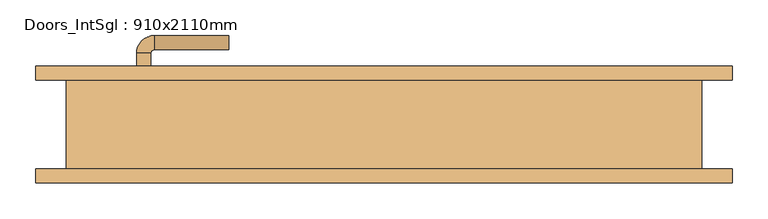
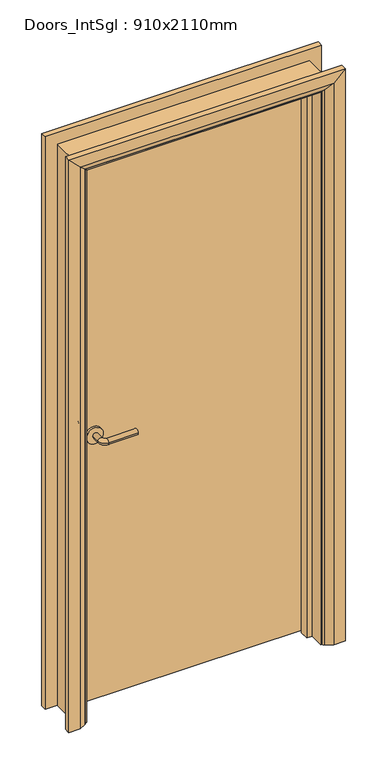
"""IFC4 building model written with IfcOpenShell, lengths in millimetres: door geometry, Doors_IntSgl : 910x2110mm."""

import ifcopenshell
import ifcopenshell.guid

model = None  # the IFC model being written
_history = None  # IfcOwnerHistory: only IFC2X3 demands one
_inside = {}  # id of a spatial element -> (the spatial element, [elements in it])
_under = {}  # id of a project, library or spatial element -> (it, [spatial elements below it])
_declared = {}  # id of a project -> (the project, [libraries it declares])
_typed = {}  # id of a type object -> (the type object, [elements of that type])
_made_of = {}  # id of a material, layer set ... -> (it, [elements and type objects made of it])


def new_model(schema):
    """Start an empty IFC model of exactly this schema.

    Asked for "IFC4X3", IfcOpenShell would pick the latest addendum, in which some entities
    have other attributes; the version numbers below select the first issue.
    IFC2X3 requires an IfcOwnerHistory on every rooted entity: one is made here for all.
    """
    global model, _history
    if schema == "IFC4X3":
        model = ifcopenshell.file(schema_version=(4, 3, 0, 0))
    else:
        model = ifcopenshell.file(schema=schema)
    _inside.clear()
    _under.clear()
    _declared.clear()
    _typed.clear()
    _made_of.clear()
    _history = None
    if model.schema == "IFC2X3":
        org = make("IfcOrganization", Name="unknown")
        user = make(
            "IfcPersonAndOrganization",
            ThePerson=make("IfcPerson", FamilyName="unknown"),
            TheOrganization=org,
        )
        app = make(
            "IfcApplication",
            ApplicationDeveloper=org,
            Version="unknown",
            ApplicationFullName="unknown",
            ApplicationIdentifier="unknown",
        )
        _history = make(
            "IfcOwnerHistory",
            OwningUser=user,
            OwningApplication=app,
            ChangeAction="ADDED",
            CreationDate=0,
        )
    return model


def make(cls, **values):
    """One entity of the class cls with the attributes given. An attribute that is None is left unset."""
    return model.create_entity(
        cls, **{name: value for name, value in values.items() if value is not None}
    )


def rooted(cls, **values):
    """An entity with a GlobalId (a new one), such as an element, a storey or a relation."""
    return make(cls, GlobalId=ifcopenshell.guid.new(), OwnerHistory=_history, **values)


def si_unit(unit_type, name, prefix=None):
    """IfcSIUnit, for example si_unit("LENGTHUNIT", "METRE", prefix="MILLI")."""
    return make("IfcSIUnit", UnitType=unit_type, Prefix=prefix, Name=name)


def assignment(units):
    """IfcUnitAssignment: the units of a project."""
    return None if units is None else make("IfcUnitAssignment", Units=units)


def point(xyz):
    """IfcCartesianPoint."""
    return None if xyz is None else make("IfcCartesianPoint", Coordinates=xyz)


def direction(xyz):
    """IfcDirection."""
    return None if xyz is None else make("IfcDirection", DirectionRatios=xyz)


def frame(location, z_axis=None, x_axis=None):
    """IfcAxis2Placement3D, a coordinate frame: its origin and axes. An axis left out is left unset."""
    return make(
        "IfcAxis2Placement3D",
        Location=point(location),
        Axis=direction(z_axis),
        RefDirection=direction(x_axis),
    )


def frame_2d(location, x_axis=None):
    """IfcAxis2Placement2D, a coordinate frame in the plane: its origin and x axis."""
    return make(
        "IfcAxis2Placement2D", Location=point(location), RefDirection=direction(x_axis)
    )


def origin():
    """The frame at (0, 0, 0) with its axes left unset."""
    return frame((0.0, 0.0, 0.0))


def place(relative_to, where):
    """IfcLocalPlacement: puts the frame where relative to a parent placement (None: the world)."""
    return make(
        "IfcLocalPlacement", PlacementRelTo=relative_to, RelativePlacement=where
    )


def context(
    kind, dimensions, precision=None, world=None, true_north=None, identifier=None
):
    """IfcGeometricRepresentationContext, for example the 3D "Model" context."""
    return make(
        "IfcGeometricRepresentationContext",
        ContextIdentifier=identifier,
        ContextType=kind,
        CoordinateSpaceDimension=dimensions,
        Precision=precision,
        WorldCoordinateSystem=world,
        TrueNorth=true_north,
    )


def project(units=None, contexts=None):
    """IfcProject with its units and contexts."""
    return rooted(
        "IfcProject",
        Name="project",
        RepresentationContexts=contexts,
        UnitsInContext=assignment(units),
    )


def spatial(cls, under=None, at=None, **own):
    """A site, building, storey or space (cls), placed at a placement, below another one or the project."""
    s = rooted(cls, ObjectPlacement=at, **own)
    if under is not None:
        _under.setdefault(under.id(), (under, []))[1].append(s)
    return s


def polyline(points):
    """IfcPolyline through the points."""
    return make("IfcPolyline", Points=[point(p) for p in points])


def circle_curve(where, radius):
    """IfcCircle in the frame where."""
    return make("IfcCircle", Position=where, Radius=radius)


def ellipse_curve(where, semi_axis1, semi_axis2):
    """IfcEllipse in the frame where."""
    return make(
        "IfcEllipse", Position=where, SemiAxis1=semi_axis1, SemiAxis2=semi_axis2
    )


def trimmed(basis, trim1, trim2, sense, master):
    """IfcTrimmedCurve: the piece of a basis curve between two trims."""
    return make(
        "IfcTrimmedCurve",
        BasisCurve=basis,
        Trim1=trim1,
        Trim2=trim2,
        SenseAgreement=sense,
        MasterRepresentation=master,
    )


def segment(curve, same_sense, transition):
    """IfcCompositeCurveSegment."""
    return make(
        "IfcCompositeCurveSegment",
        Transition=transition,
        SameSense=same_sense,
        ParentCurve=curve,
    )


def composite_curve(segments, self_intersect=None):
    """IfcCompositeCurve: segments joined end to end."""
    return make("IfcCompositeCurve", Segments=segments, SelfIntersect=self_intersect)


def outline(outer, holes=None, kind="AREA"):
    """IfcArbitraryClosedProfileDef: a profile drawn as a closed curve; with holes, ...WithVoids."""
    if holes is None:
        return make("IfcArbitraryClosedProfileDef", ProfileType=kind, OuterCurve=outer)
    return make(
        "IfcArbitraryProfileDefWithVoids",
        ProfileType=kind,
        OuterCurve=outer,
        InnerCurves=holes,
    )


def extrude(swept, where, along, depth):
    """IfcExtrudedAreaSolid: the profile swept, set in the frame where, extruded along a direction by depth."""
    return make(
        "IfcExtrudedAreaSolid",
        SweptArea=swept,
        Position=where,
        ExtrudedDirection=direction(along),
        Depth=depth,
    )


def faces_of(points, faces, orient=None, outer=None):
    """IfcFace entities. A face is a list of loops; a loop is a list of indices into points, from 0.

    orient and outer hold one flag for each loop. By default every Orientation is true, the
    first loop of a face is its IfcFaceOuterBound and the others are IfcFaceBound.
    """
    made = []
    for i, loops in enumerate(faces):
        bounds = []
        for j, loop in enumerate(loops):
            is_outer = j == 0 if outer is None else outer[i][j]
            bounds.append(
                make(
                    "IfcFaceOuterBound" if is_outer else "IfcFaceBound",
                    Bound=make("IfcPolyLoop", Polygon=[points[k] for k in loop]),
                    Orientation=True if orient is None else orient[i][j],
                )
            )
        made.append(make("IfcFace", Bounds=bounds))
    return made


def faceted_brep(points, faces, orient=None, outer=None, voids=None):
    """IfcFacetedBrep: a solid bounded by flat faces; with voids (closed shells), ...WithVoids."""
    shared = [point(p) for p in points]
    hull = make("IfcClosedShell", CfsFaces=faces_of(shared, faces, orient, outer))
    if voids is None:
        return make("IfcFacetedBrep", Outer=hull)
    return make(
        "IfcFacetedBrepWithVoids",
        Outer=hull,
        Voids=[
            make(cls, CfsFaces=faces_of(shared, fs, o, b)) for cls, fs, o, b in voids
        ],
    )


def shape(context_of_items, identifier, shape_type, items):
    """IfcShapeRepresentation: the items that make up one representation, for example the "Body"."""
    return make(
        "IfcShapeRepresentation",
        ContextOfItems=context_of_items,
        RepresentationIdentifier=identifier,
        RepresentationType=shape_type,
        Items=items,
    )


def source(mapping_origin, context_of_items, identifier, shape_type, items):
    """IfcRepresentationMap: a shape defined once, which mapped items show again and again."""
    return make(
        "IfcRepresentationMap",
        MappingOrigin=mapping_origin,
        MappedRepresentation=shape(context_of_items, identifier, shape_type, items),
    )


def transform(
    local_origin,
    x_axis=None,
    y_axis=None,
    z_axis=None,
    scale=None,
    scale2=None,
    scale3=None,
    uniform=True,
):
    """IfcCartesianTransformationOperator3D, or its non-uniform kind. x_axis, y_axis, z_axis: its Axis1, 2, 3."""
    if uniform:
        return make(
            "IfcCartesianTransformationOperator3D",
            Axis1=direction(x_axis),
            Axis2=direction(y_axis),
            LocalOrigin=point(local_origin),
            Scale=scale,
            Axis3=direction(z_axis),
        )
    return make(
        "IfcCartesianTransformationOperator3DnonUniform",
        Axis1=direction(x_axis),
        Axis2=direction(y_axis),
        LocalOrigin=point(local_origin),
        Scale=scale,
        Axis3=direction(z_axis),
        Scale2=scale2,
        Scale3=scale3,
    )


def mapped(mapping_source, mapping_target):
    """IfcMappedItem: shows the shape of a source again, moved by a transform."""
    return make(
        "IfcMappedItem", MappingSource=mapping_source, MappingTarget=mapping_target
    )


def made_of(thing, what):
    """Note that an element or type object is made of a material, layer set ...; save() writes the relation."""
    if what is not None:
        _made_of.setdefault(what.id(), (what, []))[1].append(thing)
    return thing


def element(
    cls,
    number,
    at=None,
    inside=None,
    cuts=None,
    type_object=None,
    material=None,
    context=None,
    identifier="Body",
    shape_type=None,
    held_by="IfcProductDefinitionShape",
    body=None,
    shapes=None,
    **own,
):
    """One element of the class cls, such as IfcWall. Its Tag is "e" and its number.

    at: its placement. inside: the storey or other place that contains it. cuts: it is an
    opening in that element (IfcRelVoidsElement). A single representation is given by context,
    identifier, shape_type and body (its items); several are given by shapes. held_by: the class
    of the entity that holds the representations. save() writes the other relations.
    """
    e = rooted(cls, Tag="e%d" % number, ObjectPlacement=at, **own)
    if body is not None:
        shapes = [shape(context, identifier, shape_type, body)]
    if shapes is not None:
        e.Representation = make(held_by, Representations=shapes)
    if inside is not None:
        _inside.setdefault(inside.id(), (inside, []))[1].append(e)
    if cuts is not None:
        rooted(
            "IfcRelVoidsElement", RelatingBuildingElement=cuts, RelatedOpeningElement=e
        )
    if type_object is not None:
        _typed.setdefault(type_object.id(), (type_object, []))[1].append(e)
    return made_of(e, material)


def aggregate(whole, parts):
    """IfcRelAggregates: a whole, such as a stair, and the parts it consists of."""
    return rooted("IfcRelAggregates", RelatingObject=whole, RelatedObjects=parts)


def save(model, path):
    """Write the relations noted so far, then the file.

    IfcRelAggregates (storeys below a building ...), IfcRelContainedInSpatialStructure (elements
    in a storey), IfcRelDefinesByType, IfcRelAssociatesMaterial and IfcRelDeclares: one each for
    every whole, place, type object, material and project.
    """
    for whole, parts in _under.values():
        aggregate(whole, parts)
    for where, things in _inside.values():
        rooted(
            "IfcRelContainedInSpatialStructure",
            RelatedElements=things,
            RelatingStructure=where,
        )
    for kind, things in _typed.values():
        rooted("IfcRelDefinesByType", RelatedObjects=things, RelatingType=kind)
    for what, things in _made_of.values():
        rooted("IfcRelAssociatesMaterial", RelatedObjects=things, RelatingMaterial=what)
    for by, libraries in _declared.values():
        rooted("IfcRelDeclares", RelatingContext=by, RelatedDefinitions=libraries)
    model.write(path)


def plane_surface(at):
    """IfcPlane: the flat surface through the origin of the frame at, square to its z axis."""
    return make("IfcPlane", Position=at)


def cylinder_surface(at, radius):
    """IfcCylindricalSurface: all points at the distance radius from the z axis of the frame at."""
    return make("IfcCylindricalSurface", Position=at, Radius=radius)


def revolved_surface(curve, axis_point, axis_direction):
    """IfcSurfaceOfRevolution: the curve turned about the line through axis_point along axis_direction."""
    return make(
        "IfcSurfaceOfRevolution",
        SweptCurve=make("IfcArbitraryOpenProfileDef", ProfileType="CURVE", Curve=curve),
        AxisPosition=make("IfcAxis1Placement", Location=point(axis_point), Axis=direction(axis_direction)),
    )


def advanced_brep(points, edges, surfaces, faces):
    """IfcAdvancedBrep: a solid bounded by faces that lie on surfaces and meet in shared edges.

    An edge is (start, end): straight between two places in points (the first is 0);
    or (start, end, curve); or (start, end, curve, False) where it runs against its curve.
    A face is (place in surfaces, loops), or (place, loops, False) where it looks against
    its surface's normal. A loop lists edges by number (the first is 1), with a minus sign
    where the edge is run from its end to its start. The first loop is the outer one.
    """
    corners = [point(p) for p in points]
    vertices = [make("IfcVertexPoint", VertexGeometry=c) for c in corners]
    made = []
    for start, end, *more in edges:
        made.append(
            make(
                "IfcEdgeCurve",
                EdgeStart=vertices[start],
                EdgeEnd=vertices[end],
                EdgeGeometry=more[0] if more else make("IfcPolyline", Points=[corners[start], corners[end]]),
                SameSense=more[1] if len(more) > 1 else True,
            )
        )
    hull = []
    for where, loops, *sense in faces:
        bounds = []
        for j, loop in enumerate(loops):
            ring = [make("IfcOrientedEdge", EdgeElement=made[abs(k) - 1], Orientation=k > 0) for k in loop]
            bounds.append(
                make(
                    "IfcFaceOuterBound" if j == 0 else "IfcFaceBound",
                    Bound=make("IfcEdgeLoop", EdgeList=ring),
                    Orientation=True,
                )
            )
        hull.append(make("IfcAdvancedFace", Bounds=bounds, FaceSurface=surfaces[where], SameSense=sense[0] if sense else True))
    return make("IfcAdvancedBrep", Outer=make("IfcClosedShell", CfsFaces=hull))


def doors_intsgl_910x2110mm_1208da3b(model_context):
    return source(origin(), model_context, "Body", "SolidModel", [
        advanced_brep(
        [(-348.0, 16.5, 1000.0), (-328.0, 16.5, 1000.0), (-328.0, -13.5, 1000.0), (-348.0, -13.5, 1000.0), (-323.0, -18.5, 1000.0), (-323.0, -38.5, 1000.0), (-218.0, -38.5, 1000.0), (-218.0, -18.5, 1000.0)],
        [
            (0, 1, circle_curve(frame((-338.0, 16.5, 1000.0), z_axis=(0.0, 1.0, 0.0), x_axis=(1.0, 0.0, 0.0)), 10.0)),
            (1, 0, circle_curve(frame((-338.0, 16.5, 1000.0), z_axis=(0.0, 1.0, 0.0), x_axis=(1.0, 0.0, 0.0)), 10.0)),
            (1, 2),
            (2, 3, circle_curve(frame((-338.0, -13.5, 1000.0), z_axis=(0.0, 1.0, 0.0), x_axis=(1.0, 0.0, 0.0)), 10.0)),
            (3, 0),
            (3, 2, circle_curve(frame((-338.0, -13.5, 1000.0), z_axis=(0.0, 1.0, 0.0), x_axis=(1.0, 0.0, 0.0)), 10.0)),
            (4, 5, circle_curve(frame((-323.0, -28.5, 1000.0), z_axis=(-1.0, 0.0, 0.0), x_axis=(0.0, 1.0, 0.0)), 10.0)),
            (5, 3, circle_curve(frame((-323.0, -13.5, 1000.0), z_axis=(0.0, 0.0, -1.0), x_axis=(-1.0, 0.0, 0.0)), 25.0)),
            (2, 4, circle_curve(frame((-323.0, -13.5, 1000.0), z_axis=(0.0, 0.0, 1.0), x_axis=(-1.0, 0.0, 0.0)), 5.0)),
            (5, 4, circle_curve(frame((-323.0, -28.5, 1000.0), z_axis=(-1.0, 0.0, 0.0), x_axis=(0.0, 1.0, 0.0)), 10.0)),
            (6, 7, circle_curve(frame((-218.0, -28.5, 1000.0), z_axis=(1.0, 0.0, 0.0), x_axis=(0.0, 1.0, 0.0)), 10.0)),
            (7, 6, circle_curve(frame((-218.0, -28.5, 1000.0), z_axis=(1.0, 0.0, 0.0), x_axis=(0.0, 1.0, 0.0)), 10.0)),
            (4, 7),
            (6, 5),
        ],
        [
            plane_surface(frame((-338.0, 16.5, 1000.0), z_axis=(0.0, 1.0, 0.0), x_axis=(0.0, 0.0, 1.0))),
            cylinder_surface(frame((-338.0, 16.5, 1000.0), z_axis=(0.0, 1.0, 0.0), x_axis=(1.0, 0.0, 0.0)), 10.0),
            revolved_surface(trimmed(ellipse_curve(frame((-338.0, -13.5, 1000.0), z_axis=(0.0, -1.0, 0.0), x_axis=(1.0, 0.0, 0.0)), 10.0, 10.0), [point((-348.0, -13.5, 1000.0))], [point((-328.0, -13.5, 1000.0))], True, "CARTESIAN"), (-323.0, -13.5, 1000.0), (0.0, 0.0, -1.0)),
            revolved_surface(trimmed(ellipse_curve(frame((-338.0, -13.5, 1000.0), z_axis=(0.0, -1.0, 0.0), x_axis=(1.0, 0.0, 0.0)), 10.0, 10.0), [point((-328.0, -13.5, 1000.0))], [point((-348.0, -13.5, 1000.0))], True, "CARTESIAN"), (-323.0, -13.5, 1000.0), (0.0, 0.0, -1.0)),
            plane_surface(frame((-218.0, -28.5, 1000.0), z_axis=(1.0, 0.0, 0.0), x_axis=(0.0, 0.0, 1.0))),
            cylinder_surface(frame((-323.0, -28.5, 1000.0), z_axis=(-1.0, 0.0, 0.0), x_axis=(0.0, 1.0, 0.0)), 10.0),
        ],
        [
            (0, [[1, 2]]),
            (1, [[3, 4, 5, -2]]),
            (1, [[-5, 6, -3, -1]]),
            (2, [[7, 8, -4, 9]]),
            (3, [[10, -9, -6, -8]]),
            (4, [[11, 12]]),
            (5, [[13, -11, 14, -7]]),
            (5, [[-14, -12, -13, -10]]),
        ],
    ),
        extrude(outline(composite_curve([segment(trimmed(circle_curve(frame_2d((1000.0, -340.5)), 30.0), [point((1000.0, -370.5))], [point((1000.0, -310.5))], False, "CARTESIAN"), True, "CONTINUOUS"), segment(trimmed(circle_curve(frame_2d((1000.0, -340.5)), 30.0), [point((1000.0, -310.5))], [point((1000.0, -370.5))], False, "CARTESIAN"), True, "CONTINUOUS")], self_intersect=False)), frame((0.0, 16.5, 0.0), z_axis=(0.0, 1.0, 0.0), x_axis=(0.0, 0.0, 1.0)), (0.0, 0.0, 1.0), 8.0),
        advanced_brep(
        [(-348.0, 70.5, 1000.0), (-328.0, 70.5, 1000.0), (-348.0, 100.5, 1000.0), (-328.0, 100.5, 1000.0), (-323.0, 105.5, 1000.0), (-323.0, 125.5, 1000.0), (-218.0, 125.5, 1000.0), (-218.0, 105.5, 1000.0)],
        [
            (0, 1, circle_curve(frame((-338.0, 70.5, 1000.0), z_axis=(0.0, -1.0, 0.0), x_axis=(1.0, 0.0, 0.0)), 10.0)),
            (1, 0, circle_curve(frame((-338.0, 70.5, 1000.0), z_axis=(0.0, -1.0, 0.0), x_axis=(1.0, 0.0, 0.0)), 10.0)),
            (0, 2),
            (2, 3, circle_curve(frame((-338.0, 100.5, 1000.0), z_axis=(0.0, -1.0, 0.0), x_axis=(1.0, 0.0, 0.0)), 10.0)),
            (3, 1),
            (3, 2, circle_curve(frame((-338.0, 100.5, 1000.0), z_axis=(0.0, -1.0, 0.0), x_axis=(1.0, 0.0, 0.0)), 10.0)),
            (4, 3, circle_curve(frame((-323.0, 100.5, 1000.0), z_axis=(0.0, 0.0, 1.0), x_axis=(-1.0, 0.0, 0.0)), 5.0)),
            (2, 5, circle_curve(frame((-323.0, 100.5, 1000.0), z_axis=(0.0, 0.0, -1.0), x_axis=(-1.0, 0.0, 0.0)), 25.0)),
            (5, 4, circle_curve(frame((-323.0, 115.5, 1000.0), z_axis=(-1.0, 0.0, 0.0), x_axis=(0.0, -1.0, 0.0)), 10.0)),
            (4, 5, circle_curve(frame((-323.0, 115.5, 1000.0), z_axis=(-1.0, 0.0, 0.0), x_axis=(0.0, -1.0, 0.0)), 10.0)),
            (6, 7, circle_curve(frame((-218.0, 115.5, 1000.0), z_axis=(1.0, 0.0, 0.0), x_axis=(0.0, -1.0, 0.0)), 10.0)),
            (7, 6, circle_curve(frame((-218.0, 115.5, 1000.0), z_axis=(1.0, 0.0, 0.0), x_axis=(0.0, -1.0, 0.0)), 10.0)),
            (5, 6),
            (7, 4),
        ],
        [
            plane_surface(frame((-338.0, 70.5, 1000.0), z_axis=(0.0, -1.0, 0.0), x_axis=(0.0, 0.0, 1.0))),
            cylinder_surface(frame((-338.0, 70.5, 1000.0), z_axis=(0.0, -1.0, 0.0), x_axis=(1.0, 0.0, 0.0)), 10.0),
            revolved_surface(trimmed(ellipse_curve(frame((-338.0, 100.5, 1000.0), z_axis=(0.0, -1.0, 0.0), x_axis=(1.0, 0.0, 0.0)), 10.0, 10.0), [point((-348.0, 100.5, 1000.0))], [point((-328.0, 100.5, 1000.0))], True, "CARTESIAN"), (-323.0, 100.5, 1000.0), (0.0, 0.0, -1.0)),
            revolved_surface(trimmed(ellipse_curve(frame((-338.0, 100.5, 1000.0), z_axis=(0.0, -1.0, 0.0), x_axis=(1.0, 0.0, 0.0)), 10.0, 10.0), [point((-328.0, 100.5, 1000.0))], [point((-348.0, 100.5, 1000.0))], True, "CARTESIAN"), (-323.0, 100.5, 1000.0), (0.0, 0.0, -1.0)),
            plane_surface(frame((-218.0, 115.5, 1000.0), z_axis=(1.0, 0.0, 0.0), x_axis=(0.0, 0.0, 1.0))),
            cylinder_surface(frame((-323.0, 115.5, 1000.0), z_axis=(-1.0, 0.0, 0.0), x_axis=(0.0, -1.0, 0.0)), 10.0),
        ],
        [
            (0, [[1, 2]]),
            (1, [[-1, 3, 4, 5]]),
            (1, [[-2, -5, 6, -3]]),
            (2, [[7, -4, 8, 9]]),
            (3, [[-8, -6, -7, 10]]),
            (4, [[11, 12]]),
            (5, [[-9, 13, -12, 14]]),
            (5, [[-10, -14, -11, -13]]),
        ],
    ),
        extrude(outline(composite_curve([segment(trimmed(circle_curve(frame_2d((1000.0, -340.5)), 30.0), [point((1000.0, -370.5))], [point((1000.0, -310.5))], False, "CARTESIAN"), True, "CONTINUOUS"), segment(trimmed(circle_curve(frame_2d((1000.0, -340.5)), 30.0), [point((1000.0, -310.5))], [point((1000.0, -370.5))], False, "CARTESIAN"), True, "CONTINUOUS")], self_intersect=False)), frame((0.0, 62.5, 0.0), z_axis=(0.0, 1.0, 0.0), x_axis=(0.0, 0.0, 1.0)), (0.0, 0.0, 1.0), 8.0),
        extrude(outline(polyline([(413.0, 24.5), (-413.0, 24.5), (-413.0, 62.5), (413.0, 62.5), (413.0, 24.5)])), frame((0.0, 0.0, 8.0), z_axis=(0.0, 0.0, 1.0), x_axis=(1.0, 0.0, 0.0)), (0.0, 0.0, 1.0), 2060.0),
        advanced_brep(
        [(490.0, 82.5, 0.0), (490.0, 62.5, 0.0), (420.0, 62.5, 0.0), (424.0, 68.5, 0.0), (450.0, 82.5, 0.0), (490.0, 82.5, 2145.0), (490.0, 62.5, 2145.0), (-490.0, 62.5, 2145.0), (-490.0, 62.5, 0.0), (-420.0, 62.5, 0.0), (-420.0, 62.5, 2075.0), (420.0, 62.5, 2075.0), (424.0, 68.5, 2079.0), (450.0, 82.5, 2105.0), (-450.0, 82.5, 2105.0), (-450.0, 82.5, 0.0), (-490.0, 82.5, 0.0), (-490.0, 82.5, 2145.0), (-424.0, 68.5, 2079.0), (-424.0, 68.5, 0.0)],
        [
            (0, 1),
            (1, 2),
            (2, 3, circle_curve(frame((428.0, 61.5, 0.0), z_axis=(0.0, 0.0, -1.0), x_axis=(1.0, 0.0, 0.0)), 8.0622577)),
            (3, 4),
            (4, 0),
            (0, 5),
            (5, 6),
            (6, 1),
            (6, 7),
            (7, 8),
            (8, 9),
            (9, 10),
            (10, 11),
            (11, 2),
            (11, 12, ellipse_curve(frame((428.0, 61.5, 2083.0), z_axis=(0.7071067811865475, 0.0, -0.7071067811865475), x_axis=(-0.7071067811865474, 0.0, -0.7071067811865476)), 11.4017543, 8.0622577)),
            (12, 3),
            (12, 13),
            (13, 4),
            (13, 14),
            (14, 15),
            (15, 16),
            (16, 17),
            (17, 5),
            (17, 7),
            (10, 18, ellipse_curve(frame((-428.0, 61.5, 2083.0), z_axis=(0.7071067811865475, 0.0, 0.7071067811865475), x_axis=(0.7071067811865476, 0.0, -0.7071067811865474)), 11.4017543, 8.0622577)),
            (18, 12),
            (18, 14),
            (15, 19),
            (19, 9, circle_curve(frame((-428.0, 61.5, 0.0), z_axis=(0.0, 0.0, -1.0), x_axis=(-1.0, 0.0, 0.0)), 8.0622577)),
            (8, 16),
            (19, 18),
        ],
        [
            plane_surface(frame((420.0, 62.5, 0.0), z_axis=(0.0, 0.0, -1.0), x_axis=(0.0, -1.0, 0.0))),
            plane_surface(frame((490.0, 82.5, 0.0), z_axis=(1.0, 0.0, 0.0), x_axis=(0.0, 0.0, 1.0))),
            plane_surface(frame((490.0, 62.5, 0.0), z_axis=(0.0, -1.0, 0.0), x_axis=(0.0, 0.0, 1.0))),
            cylinder_surface(frame((428.0, 61.5, 0.0), z_axis=(0.0, 0.0, -1.0), x_axis=(1.0, 0.0, 0.0)), 8.0622577),
            plane_surface(frame((424.0, 68.5, 0.0), z_axis=(-0.4740998230350126, 0.880471099922178, 0.0), x_axis=(0.0, 0.0, 1.0))),
            plane_surface(frame((450.0, 82.5, 0.0), z_axis=(0.0, 1.0, 0.0), x_axis=(0.0, 0.0, 1.0))),
            plane_surface(frame((490.0, 82.5, 2145.0), z_axis=(0.0, 0.0, 1.0), x_axis=(-1.0, 0.0, 0.0))),
            cylinder_surface(frame((420.0, 61.5, 2083.0), z_axis=(1.0, 0.0, 0.0), x_axis=(0.0, 0.0, 1.0)), 8.0622577),
            plane_surface(frame((424.0, 68.5, 2079.0), z_axis=(0.0, 0.8804710999221764, -0.4740998230350154), x_axis=(-1.0, 0.0, 0.0))),
            plane_surface(frame((-420.0, 62.5, 0.0), z_axis=(0.0, 0.0, -1.0), x_axis=(0.0, -1.0, 0.0))),
            plane_surface(frame((-490.0, 82.5, 2145.0), z_axis=(-1.0, 0.0, 0.0), x_axis=(0.0, 0.0, -1.0))),
            cylinder_surface(frame((-428.0, 61.5, 2075.0), z_axis=(0.0, 0.0, 1.0), x_axis=(-1.0, 0.0, 0.0)), 8.0622577),
            plane_surface(frame((-424.0, 68.5, 2079.0), z_axis=(0.47409982303501824, 0.8804710999221749, 0.0), x_axis=(0.0, 0.0, -1.0))),
        ],
        [
            (0, [[1, 2, 3, 4, 5]]),
            (1, [[-1, 6, 7, 8]]),
            (2, [[-2, -8, 9, 10, 11, 12, 13, 14]]),
            (3, [[-3, -14, 15, 16]]),
            (4, [[-4, -16, 17, 18]]),
            (5, [[-5, -18, 19, 20, 21, 22, 23, -6]]),
            (6, [[-7, -23, 24, -9]]),
            (7, [[-15, -13, 25, 26]]),
            (8, [[-17, -26, 27, -19]]),
            (9, [[-21, 28, 29, -11, 30]]),
            (10, [[-24, -22, -30, -10]]),
            (11, [[-25, -12, -29, 31]]),
            (12, [[-27, -31, -28, -20]]),
        ],
    ),
        extrude(outline(polyline([(0.0, -415.0), (0.0, -396.0), (2051.0, -396.0), (2051.0, 396.0), (0.0, 396.0), (0.0, 415.0), (2070.0, 415.0), (2070.0, -415.0), (0.0, -415.0)])), frame((0.0, -9.5, 0.0), z_axis=(0.0, 1.0, 0.0), x_axis=(0.0, 0.0, 1.0)), (0.0, 0.0, 1.0), 32.0),
        advanced_brep(
        [(-490.0, -82.5, 0.0), (-490.0, -62.5, 0.0), (-420.0, -62.5, 0.0), (-424.0, -68.5, 0.0), (-450.0, -82.5, 0.0), (-490.0, -82.5, 2145.0), (-490.0, -62.5, 2145.0), (-420.0, -62.5, 2075.0), (-424.0, -68.5, 2079.0), (-450.0, -82.5, 2105.0), (490.0, -82.5, 2145.0), (490.0, -62.5, 2145.0), (420.0, -62.5, 2075.0), (424.0, -68.5, 2079.0), (450.0, -82.5, 2105.0), (490.0, -82.5, 0.0), (450.0, -82.5, 0.0), (424.0, -68.5, 0.0), (420.0, -62.5, 0.0), (490.0, -62.5, 0.0)],
        [
            (0, 1),
            (1, 2),
            (2, 3, circle_curve(frame((-428.0, -61.5, 0.0), z_axis=(0.0, 0.0, -1.0), x_axis=(-1.0, 0.0, 0.0)), 8.0622577)),
            (3, 4),
            (4, 0),
            (0, 5),
            (5, 6),
            (6, 1),
            (6, 7),
            (7, 2),
            (7, 8, ellipse_curve(frame((-428.0, -61.5, 2083.0), z_axis=(-0.7071067811865475, 0.0, -0.7071067811865475), x_axis=(0.7071067811865474, 0.0, -0.7071067811865476)), 11.4017543, 8.0622577)),
            (8, 3),
            (8, 9),
            (9, 4),
            (9, 5),
            (5, 10),
            (10, 11),
            (11, 6),
            (11, 12),
            (12, 7),
            (12, 13, ellipse_curve(frame((428.0, -61.5, 2083.0), z_axis=(-0.7071067811865475, 0.0, 0.7071067811865475), x_axis=(-0.7071067811865476, 0.0, -0.7071067811865474)), 11.4017543, 8.0622577)),
            (13, 8),
            (13, 14),
            (14, 9),
            (14, 10),
            (15, 16),
            (16, 17),
            (17, 18, circle_curve(frame((428.0, -61.5, 0.0), z_axis=(0.0, 0.0, -1.0), x_axis=(1.0, 0.0, 0.0)), 8.0622577)),
            (18, 19),
            (19, 15),
            (10, 15),
            (19, 11),
            (18, 12),
            (17, 13),
            (16, 14),
        ],
        [
            plane_surface(frame((-420.0, -135.3010989, 0.0), z_axis=(0.0, 0.0, -1.0), x_axis=(1.0, 0.0, 0.0))),
            plane_surface(frame((-490.0, -82.5, 0.0), z_axis=(-1.0, 0.0, 0.0), x_axis=(0.0, 0.0, 1.0))),
            plane_surface(frame((-490.0, -62.5, 0.0), z_axis=(0.0, 1.0, 0.0), x_axis=(0.0, 0.0, 1.0))),
            cylinder_surface(frame((-428.0, -61.5, 0.0), z_axis=(0.0, 0.0, -1.0), x_axis=(-1.0, 0.0, 0.0)), 8.0622577),
            plane_surface(frame((-424.0, -68.5, 0.0), z_axis=(0.4740998230350183, -0.8804710999221749, 0.0), x_axis=(0.0, 0.0, 1.0))),
            plane_surface(frame((-450.0, -82.5, 0.0), z_axis=(0.0, -1.0, 0.0), x_axis=(0.0, 0.0, 1.0))),
            plane_surface(frame((-490.0, -82.5, 2145.0), z_axis=(0.0, 0.0, 1.0), x_axis=(1.0, 0.0, 0.0))),
            plane_surface(frame((-490.0, -62.5, 2145.0), z_axis=(0.0, 1.0, 0.0), x_axis=(1.0, 0.0, 0.0))),
            cylinder_surface(frame((-420.0, -61.5, 2083.0), z_axis=(-1.0, 0.0, 0.0), x_axis=(0.0, 0.0, 1.0)), 8.0622577),
            plane_surface(frame((-424.0, -68.5, 2079.0), z_axis=(0.0, -0.8804710999221749, -0.4740998230350183), x_axis=(1.0, 0.0, 0.0))),
            plane_surface(frame((-450.0, -82.5, 2105.0), z_axis=(0.0, -1.0, 0.0), x_axis=(1.0, 0.0, 0.0))),
            plane_surface(frame((420.0, -135.3010989, 0.0), z_axis=(0.0, 0.0, -1.0), x_axis=(-1.0, 0.0, 0.0))),
            plane_surface(frame((490.0, -82.5, 2145.0), z_axis=(1.0, 0.0, 0.0), x_axis=(0.0, 0.0, -1.0))),
            plane_surface(frame((490.0, -62.5, 2145.0), z_axis=(0.0, 1.0, 0.0), x_axis=(0.0, 0.0, -1.0))),
            cylinder_surface(frame((428.0, -61.5, 2075.0), z_axis=(0.0, 0.0, 1.0), x_axis=(1.0, 0.0, 0.0)), 8.0622577),
            plane_surface(frame((424.0, -68.5, 2079.0), z_axis=(-0.4740998230350183, -0.8804710999221749, 0.0), x_axis=(0.0, 0.0, -1.0))),
            plane_surface(frame((450.0, -82.5, 2105.0), z_axis=(0.0, -1.0, 0.0), x_axis=(0.0, 0.0, -1.0))),
        ],
        [
            (0, [[1, 2, 3, 4, 5]]),
            (1, [[-1, 6, 7, 8]]),
            (2, [[-2, -8, 9, 10]]),
            (3, [[-3, -10, 11, 12]]),
            (4, [[-4, -12, 13, 14]]),
            (5, [[-5, -14, 15, -6]]),
            (6, [[-7, 16, 17, 18]]),
            (7, [[-9, -18, 19, 20]]),
            (8, [[-11, -20, 21, 22]]),
            (9, [[-13, -22, 23, 24]]),
            (10, [[-15, -24, 25, -16]]),
            (11, [[26, 27, 28, 29, 30]]),
            (12, [[-17, 31, -30, 32]]),
            (13, [[-19, -32, -29, 33]]),
            (14, [[-21, -33, -28, 34]]),
            (15, [[-23, -34, -27, 35]]),
            (16, [[-25, -35, -26, -31]]),
        ],
    ),
        faceted_brep([(-415.0, 62.5, 0.0), (-415.0, -62.5, 0.0), (-447.0, -62.5, 0.0), (-447.0, 62.5, 0.0), (-415.0, 62.5, 2070.0), (-415.0, -62.5, 2070.0), (-447.0, -62.5, 2102.0), (-447.0, 62.5, 2102.0), (415.0, 62.5, 2070.0), (415.0, -62.5, 2070.0), (447.0, -62.5, 2102.0), (447.0, 62.5, 2102.0), (415.0, 62.5, 0.0), (447.0, 62.5, 0.0), (447.0, -62.5, 0.0), (415.0, -62.5, 0.0)], [[[0, 1, 2, 3]], [[1, 0, 4, 5]], [[2, 1, 5, 6]], [[3, 2, 6, 7]], [[0, 3, 7, 4]], [[5, 4, 8, 9]], [[6, 5, 9, 10]], [[7, 6, 10, 11]], [[4, 7, 11, 8]], [[12, 13, 14, 15]], [[9, 8, 12, 15]], [[10, 9, 15, 14]], [[11, 10, 14, 13]], [[8, 11, 13, 12]]]),
    ])


if __name__ == "__main__":
    model = new_model("IFC4")
    model_context = context("Model", 3, world=origin())
    ifc_project = project(units=[si_unit("LENGTHUNIT", "METRE", prefix="MILLI")], contexts=[model_context])
    site = spatial("IfcSite", under=ifc_project)
    building = spatial("IfcBuilding", under=site)
    placement = place(None, origin())
    doors_intsgl_910x2110mm_shape = doors_intsgl_910x2110mm_1208da3b(model_context)
    element("IfcDoor", 1, ObjectType="Doors_IntSgl : 910x2110mm", at=placement, inside=building, context=model_context, shape_type="MappedRepresentation", body=[
        mapped(doors_intsgl_910x2110mm_shape, transform((0.0, 0.0, 0.0), x_axis=(1.0, 0.0, 0.0), y_axis=(0.0, 1.0, 0.0), z_axis=(0.0, 0.0, 1.0))),
    ])
    save(model, "model.ifc")

# Revit data of these elements
# Project information
#   Project Issue Date = "Issue Date"
#   Project Status = "Project Status"
#   Client Name = "PM & BIM"
#   Project Address = "Enter address here"
#   Project Name = "Assignment 1"
#   Project Number = "Project Number"
# Type "Doors_IntSgl : 910x2110mm"
#   Construction Type Id = "MDOOR"
#   Type Mark = "41"
#   Type Comments = "Internal Single"
#   Operation = "SingleSwingRight"
#   Manufacturer = "Revit"
#   Keynote = "L20"
#   Description = "Internal Single Door"
#   Analytic Construction = "Metal"
#   UnderCut = 8 mm
#   Tolerance = 2 mm
#   Thickness = 38 mm
#   Thermal Resistance (R) = 0.270117 (m²·K)/W
#   Structural Tolerance = 8 mm
#   StopDepth = 32 mm
#   Stop Thickness = 19 mm
#   Rough Width = 910 mm
#   Rough Height = 2110 mm
#   Height to Top Lock Rail = 1000 mm
#   Heat Transfer Coefficient (U) = 3.7021 W/(m²·K)
#   Handle Z Distance = 1000 mm
#   Handle X Distance = 75 mm
#   Frame Thickness = 32 mm
#   Door Panel Width = 826 mm
#   Door Panel Thickness = 38 mm
#   Door Panel Offset = 0 mm
#   Height = 2110 mm
#   Width = 910 mm
#   Door Panel Height = 2060 mm
#   Architrave Setback = 5 mm
#   Vis - Ironmongery = yes
#   Material Ironmongery = Door - Handle
#   Material Frame = Door - Frame/Mullion (1)
#   Material Door = Door - Panel
#   Material Architrave = Door - Architrave
#   Visual Light Transmittance = 0
#   Solar Heat Gain Coefficient = 0
#   Function = (empty or 0)
#   Wall Closure = (empty or 0)
# Element 1 (IfcDoor, "Doors_IntSgl : 910x2110mm")
#   Materials on its faces: "Door - Architrave", "Door - Handle", "Door - Frame/Mullion (1)", "Door - Panel"
# Materials
#   "Door - Handle": class "Miscellaneous", colour RGB 0 0 0, transparency 0, Keynote = "P21", Cost = 0
#   "Door - Frame/Mullion (1)": class "Wood", colour RGB 212 179 113, transparency 0, Keynote = "L20", Cost = 0
#   "Door - Panel": class "Wood", colour RGB 210 159 95, transparency 0, Keynote = "L20", Cost = 0
#   "Door - Architrave": class "Wood", colour RGB 154 90 5, transparency 0, Keynote = "P20", Cost = 0
